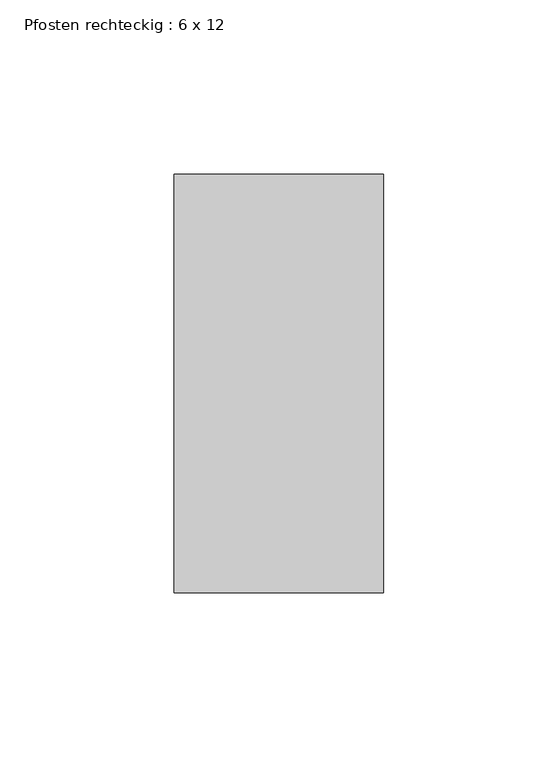
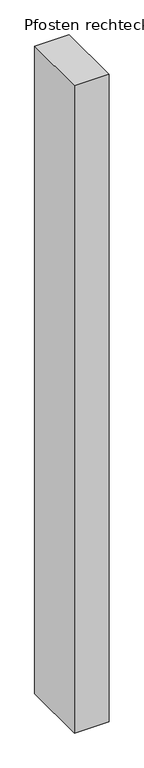
"""IFC4 building model written with IfcOpenShell, lengths in millimetres: member geometry, Pfosten rechteckig : 6 x 12."""

from ifc_helpers import new_model, si_unit, frame, origin, place, context, project, spatial, polyline, outline, extrude, source, transform, mapped, element, save


def pfosten_rechteckig_6_x_12_8bb825ca(model_context):
    return source(origin(), model_context, "Body", "SweptSolid", [
        extrude(outline(polyline([(30.0, 60.0), (30.0, -60.0), (-30.0, -60.0), (-30.0, 60.0), (30.0, 60.0)])), frame((0.0, 0.0, -1190.0), z_axis=(0.0, 0.0, 1.0), x_axis=(1.0, 0.0, 0.0)), (0.0, 0.0, 1.0), 1190.0),
    ])


if __name__ == "__main__":
    model = new_model("IFC4")
    model_context = context("Model", 3, world=origin())
    ifc_project = project(units=[si_unit("LENGTHUNIT", "METRE", prefix="MILLI")], contexts=[model_context])
    site = spatial("IfcSite", under=ifc_project)
    building = spatial("IfcBuilding", under=site)
    placement = place(None, origin())
    pfosten_rechteckig_6_x_12_shape = pfosten_rechteckig_6_x_12_8bb825ca(model_context)
    element("IfcMember", 1, ObjectType="Pfosten rechteckig : 6 x 12", at=placement, inside=building, context=model_context, shape_type="MappedRepresentation", body=[
        mapped(pfosten_rechteckig_6_x_12_shape, transform((0.0, 0.0, 0.0), x_axis=(1.0, 0.0, 0.0), y_axis=(0.0, 1.0, 0.0), z_axis=(0.0, 0.0, 1.0))),
    ])
    save(model, "model.ifc")

# Revit data of these elements
# Type "Pfosten rechteckig : 6 x 12"
#   built-in parameter 1007304 = 0.393701 (stored number, unit not read)
#   built-in parameter 1007301 = 0.0984252 (stored number, unit not read)
#   built-in parameter 1007300 = 0.0984252 (stored number, unit not read)
# Element 1 (IfcMember, "Pfosten rechteckig : 6 x 12")
#   Materials on its faces: "Metall - verzinkt"
# Materials
#   "Metall - verzinkt": class "Allgemeines", colour RGB 200 200 200, transparency 0, Cost = 0
